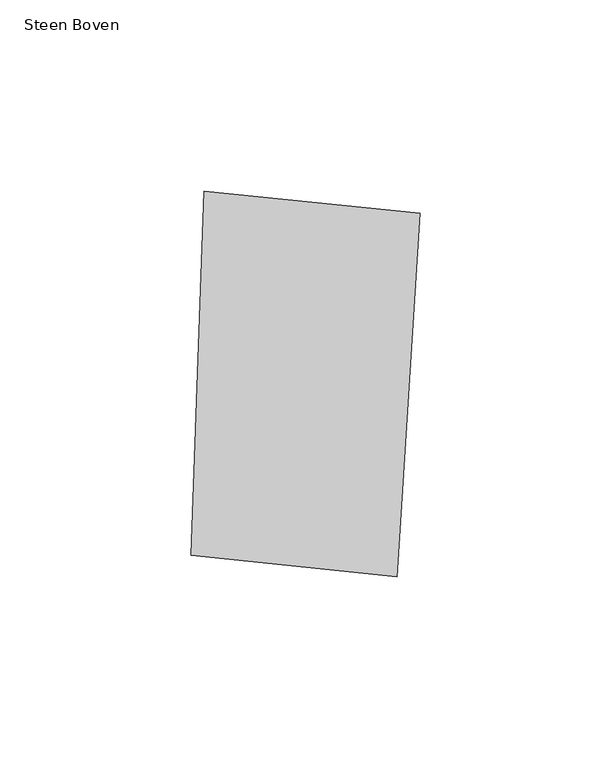
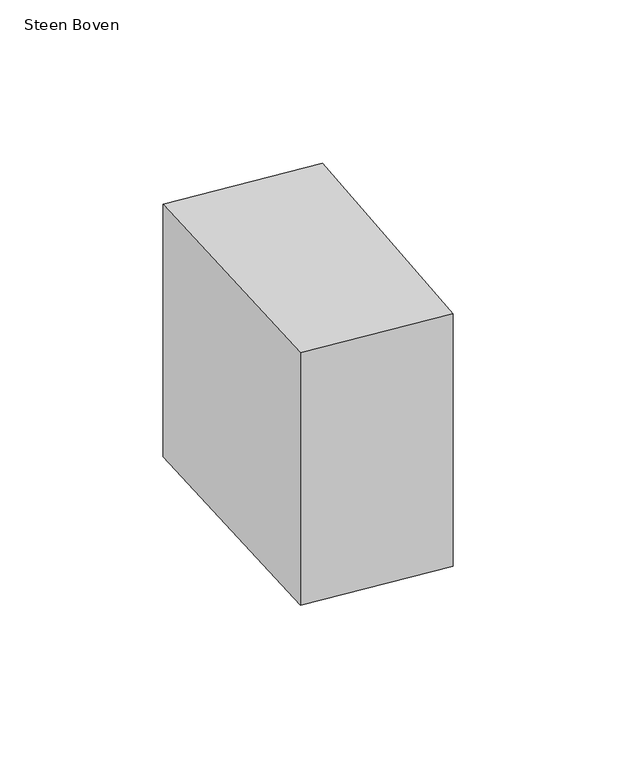
"""IFC4 building model written with IfcOpenShell, lengths in millimetres: proxy geometry, 00_GMA_steen_versie_4 : Steen Boven."""

from ifc_helpers import new_model, si_unit, origin, origin_with_axes, place, context, project, spatial, polyline, outline, extrude, source, transform, mapped, element, save


def steen_boven_b8bb974b(model_context):
    return source(origin(), model_context, "Body", "SweptSolid", [
        extrude(outline(polyline([(103.6996156, 119.0498858), (97.7707279, 24.1543987), (43.92079, 29.6806434), (47.3296437, 124.8410319), (103.6996156, 119.0498858)])), origin_with_axes(), (0.0, 0.0, 1.0), 100.0),
    ])


if __name__ == "__main__":
    model = new_model("IFC4")
    model_context = context("Model", 3, world=origin())
    ifc_project = project(units=[si_unit("LENGTHUNIT", "METRE", prefix="MILLI")], contexts=[model_context])
    site = spatial("IfcSite", under=ifc_project)
    building = spatial("IfcBuilding", under=site)
    placement = place(None, origin())
    steen_boven_shape = steen_boven_b8bb974b(model_context)
    element("IfcBuildingElementProxy", 1, Name="00_GMA_steen_versie_4 : Steen Boven", ObjectType="00_GMA_steen_versie_4 : Steen Boven", at=placement, inside=building, context=model_context, shape_type="MappedRepresentation", body=[
        mapped(steen_boven_shape, transform((0.0, 0.0, 0.0), x_axis=(1.0, 0.0, 0.0), y_axis=(0.0, 1.0, 0.0), z_axis=(0.0, 0.0, 1.0))),
    ])
    save(model, "model.ifc")

# Revit data of these elements
# Type "00_GMA_steen_versie_4 : Steen Boven"
#   StootVoegHalfBoven [instance default] = 5 mm
#   StootVoegHalf [instance default] = 5 mm
#   StootVoegBreedteOnder = 10 mm
#   StootVoegBreedteBoven = 10 mm
#   Steendikte = 100 mm
#   LintVoegOnderHalf = 5 mm
#   LintVoegOnder = 10 mm
#   LintVoegBovenHalf = 0 mm
#   LintVoegBoven = 0 mm
#   materiaal = none
#   MateriaalVoeg = none
#   Default Elevation = 0
